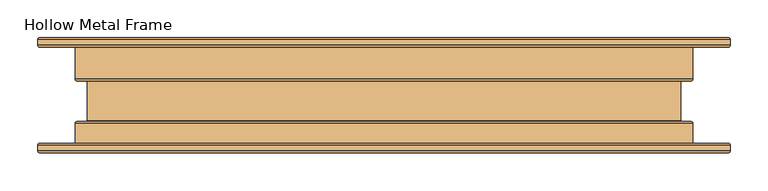
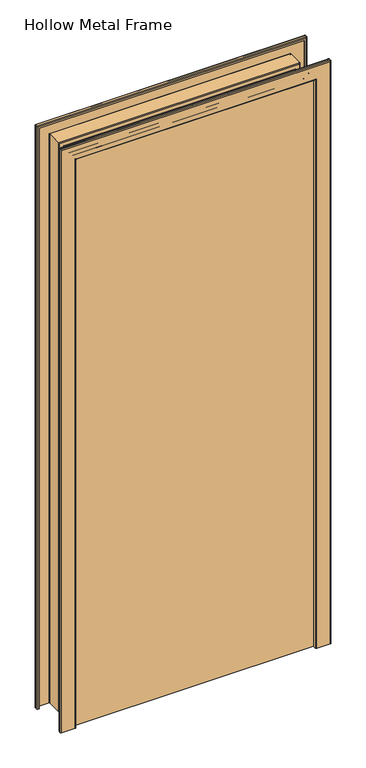
"""IFC4 building model written with IfcOpenShell, lengths in millimetres: door geometry, Hollow Metal Frame."""

import ifcopenshell
import ifcopenshell.guid

model = None  # the IFC model being written
_history = None  # IfcOwnerHistory: only IFC2X3 demands one
_inside = {}  # id of a spatial element -> (the spatial element, [elements in it])
_under = {}  # id of a project, library or spatial element -> (it, [spatial elements below it])
_declared = {}  # id of a project -> (the project, [libraries it declares])
_typed = {}  # id of a type object -> (the type object, [elements of that type])
_made_of = {}  # id of a material, layer set ... -> (it, [elements and type objects made of it])


def new_model(schema):
    """Start an empty IFC model of exactly this schema.

    Asked for "IFC4X3", IfcOpenShell would pick the latest addendum, in which some entities
    have other attributes; the version numbers below select the first issue.
    IFC2X3 requires an IfcOwnerHistory on every rooted entity: one is made here for all.
    """
    global model, _history
    if schema == "IFC4X3":
        model = ifcopenshell.file(schema_version=(4, 3, 0, 0))
    else:
        model = ifcopenshell.file(schema=schema)
    _inside.clear()
    _under.clear()
    _declared.clear()
    _typed.clear()
    _made_of.clear()
    _history = None
    if model.schema == "IFC2X3":
        org = make("IfcOrganization", Name="unknown")
        user = make(
            "IfcPersonAndOrganization",
            ThePerson=make("IfcPerson", FamilyName="unknown"),
            TheOrganization=org,
        )
        app = make(
            "IfcApplication",
            ApplicationDeveloper=org,
            Version="unknown",
            ApplicationFullName="unknown",
            ApplicationIdentifier="unknown",
        )
        _history = make(
            "IfcOwnerHistory",
            OwningUser=user,
            OwningApplication=app,
            ChangeAction="ADDED",
            CreationDate=0,
        )
    return model


def make(cls, **values):
    """One entity of the class cls with the attributes given. An attribute that is None is left unset."""
    return model.create_entity(
        cls, **{name: value for name, value in values.items() if value is not None}
    )


def rooted(cls, **values):
    """An entity with a GlobalId (a new one), such as an element, a storey or a relation."""
    return make(cls, GlobalId=ifcopenshell.guid.new(), OwnerHistory=_history, **values)


def si_unit(unit_type, name, prefix=None):
    """IfcSIUnit, for example si_unit("LENGTHUNIT", "METRE", prefix="MILLI")."""
    return make("IfcSIUnit", UnitType=unit_type, Prefix=prefix, Name=name)


def assignment(units):
    """IfcUnitAssignment: the units of a project."""
    return None if units is None else make("IfcUnitAssignment", Units=units)


def point(xyz):
    """IfcCartesianPoint."""
    return None if xyz is None else make("IfcCartesianPoint", Coordinates=xyz)


def direction(xyz):
    """IfcDirection."""
    return None if xyz is None else make("IfcDirection", DirectionRatios=xyz)


def frame(location, z_axis=None, x_axis=None):
    """IfcAxis2Placement3D, a coordinate frame: its origin and axes. An axis left out is left unset."""
    return make(
        "IfcAxis2Placement3D",
        Location=point(location),
        Axis=direction(z_axis),
        RefDirection=direction(x_axis),
    )


def origin():
    """The frame at (0, 0, 0) with its axes left unset."""
    return frame((0.0, 0.0, 0.0))


def origin_with_axes():
    """The frame at (0, 0, 0) with the z axis (0, 0, 1) and the x axis (1, 0, 0) written out."""
    return frame((0.0, 0.0, 0.0), z_axis=(0.0, 0.0, 1.0), x_axis=(1.0, 0.0, 0.0))


def place(relative_to, where):
    """IfcLocalPlacement: puts the frame where relative to a parent placement (None: the world)."""
    return make(
        "IfcLocalPlacement", PlacementRelTo=relative_to, RelativePlacement=where
    )


def context(
    kind, dimensions, precision=None, world=None, true_north=None, identifier=None
):
    """IfcGeometricRepresentationContext, for example the 3D "Model" context."""
    return make(
        "IfcGeometricRepresentationContext",
        ContextIdentifier=identifier,
        ContextType=kind,
        CoordinateSpaceDimension=dimensions,
        Precision=precision,
        WorldCoordinateSystem=world,
        TrueNorth=true_north,
    )


def project(units=None, contexts=None):
    """IfcProject with its units and contexts."""
    return rooted(
        "IfcProject",
        Name="project",
        RepresentationContexts=contexts,
        UnitsInContext=assignment(units),
    )


def spatial(cls, under=None, at=None, **own):
    """A site, building, storey or space (cls), placed at a placement, below another one or the project."""
    s = rooted(cls, ObjectPlacement=at, **own)
    if under is not None:
        _under.setdefault(under.id(), (under, []))[1].append(s)
    return s


def polyline(points):
    """IfcPolyline through the points."""
    return make("IfcPolyline", Points=[point(p) for p in points])


def circle_curve(where, radius):
    """IfcCircle in the frame where."""
    return make("IfcCircle", Position=where, Radius=radius)


def ellipse_curve(where, semi_axis1, semi_axis2):
    """IfcEllipse in the frame where."""
    return make(
        "IfcEllipse", Position=where, SemiAxis1=semi_axis1, SemiAxis2=semi_axis2
    )


def outline(outer, holes=None, kind="AREA"):
    """IfcArbitraryClosedProfileDef: a profile drawn as a closed curve; with holes, ...WithVoids."""
    if holes is None:
        return make("IfcArbitraryClosedProfileDef", ProfileType=kind, OuterCurve=outer)
    return make(
        "IfcArbitraryProfileDefWithVoids",
        ProfileType=kind,
        OuterCurve=outer,
        InnerCurves=holes,
    )


def extrude(swept, where, along, depth):
    """IfcExtrudedAreaSolid: the profile swept, set in the frame where, extruded along a direction by depth."""
    return make(
        "IfcExtrudedAreaSolid",
        SweptArea=swept,
        Position=where,
        ExtrudedDirection=direction(along),
        Depth=depth,
    )


def shape(context_of_items, identifier, shape_type, items):
    """IfcShapeRepresentation: the items that make up one representation, for example the "Body"."""
    return make(
        "IfcShapeRepresentation",
        ContextOfItems=context_of_items,
        RepresentationIdentifier=identifier,
        RepresentationType=shape_type,
        Items=items,
    )


def source(mapping_origin, context_of_items, identifier, shape_type, items):
    """IfcRepresentationMap: a shape defined once, which mapped items show again and again."""
    return make(
        "IfcRepresentationMap",
        MappingOrigin=mapping_origin,
        MappedRepresentation=shape(context_of_items, identifier, shape_type, items),
    )


def transform(
    local_origin,
    x_axis=None,
    y_axis=None,
    z_axis=None,
    scale=None,
    scale2=None,
    scale3=None,
    uniform=True,
):
    """IfcCartesianTransformationOperator3D, or its non-uniform kind. x_axis, y_axis, z_axis: its Axis1, 2, 3."""
    if uniform:
        return make(
            "IfcCartesianTransformationOperator3D",
            Axis1=direction(x_axis),
            Axis2=direction(y_axis),
            LocalOrigin=point(local_origin),
            Scale=scale,
            Axis3=direction(z_axis),
        )
    return make(
        "IfcCartesianTransformationOperator3DnonUniform",
        Axis1=direction(x_axis),
        Axis2=direction(y_axis),
        LocalOrigin=point(local_origin),
        Scale=scale,
        Axis3=direction(z_axis),
        Scale2=scale2,
        Scale3=scale3,
    )


def mapped(mapping_source, mapping_target):
    """IfcMappedItem: shows the shape of a source again, moved by a transform."""
    return make(
        "IfcMappedItem", MappingSource=mapping_source, MappingTarget=mapping_target
    )


def made_of(thing, what):
    """Note that an element or type object is made of a material, layer set ...; save() writes the relation."""
    if what is not None:
        _made_of.setdefault(what.id(), (what, []))[1].append(thing)
    return thing


def element(
    cls,
    number,
    at=None,
    inside=None,
    cuts=None,
    type_object=None,
    material=None,
    context=None,
    identifier="Body",
    shape_type=None,
    held_by="IfcProductDefinitionShape",
    body=None,
    shapes=None,
    **own,
):
    """One element of the class cls, such as IfcWall. Its Tag is "e" and its number.

    at: its placement. inside: the storey or other place that contains it. cuts: it is an
    opening in that element (IfcRelVoidsElement). A single representation is given by context,
    identifier, shape_type and body (its items); several are given by shapes. held_by: the class
    of the entity that holds the representations. save() writes the other relations.
    """
    e = rooted(cls, Tag="e%d" % number, ObjectPlacement=at, **own)
    if body is not None:
        shapes = [shape(context, identifier, shape_type, body)]
    if shapes is not None:
        e.Representation = make(held_by, Representations=shapes)
    if inside is not None:
        _inside.setdefault(inside.id(), (inside, []))[1].append(e)
    if cuts is not None:
        rooted(
            "IfcRelVoidsElement", RelatingBuildingElement=cuts, RelatedOpeningElement=e
        )
    if type_object is not None:
        _typed.setdefault(type_object.id(), (type_object, []))[1].append(e)
    return made_of(e, material)


def aggregate(whole, parts):
    """IfcRelAggregates: a whole, such as a stair, and the parts it consists of."""
    return rooted("IfcRelAggregates", RelatingObject=whole, RelatedObjects=parts)


def save(model, path):
    """Write the relations noted so far, then the file.

    IfcRelAggregates (storeys below a building ...), IfcRelContainedInSpatialStructure (elements
    in a storey), IfcRelDefinesByType, IfcRelAssociatesMaterial and IfcRelDeclares: one each for
    every whole, place, type object, material and project.
    """
    for whole, parts in _under.values():
        aggregate(whole, parts)
    for where, things in _inside.values():
        rooted(
            "IfcRelContainedInSpatialStructure",
            RelatedElements=things,
            RelatingStructure=where,
        )
    for kind, things in _typed.values():
        rooted("IfcRelDefinesByType", RelatedObjects=things, RelatingType=kind)
    for what, things in _made_of.values():
        rooted("IfcRelAssociatesMaterial", RelatedObjects=things, RelatingMaterial=what)
    for by, libraries in _declared.values():
        rooted("IfcRelDeclares", RelatingContext=by, RelatedDefinitions=libraries)
    model.write(path)


def plane_surface(at):
    """IfcPlane: the flat surface through the origin of the frame at, square to its z axis."""
    return make("IfcPlane", Position=at)


def cylinder_surface(at, radius):
    """IfcCylindricalSurface: all points at the distance radius from the z axis of the frame at."""
    return make("IfcCylindricalSurface", Position=at, Radius=radius)


def revolved_surface(curve, axis_point, axis_direction):
    """IfcSurfaceOfRevolution: the curve turned about the line through axis_point along axis_direction."""
    return make(
        "IfcSurfaceOfRevolution",
        SweptCurve=make("IfcArbitraryOpenProfileDef", ProfileType="CURVE", Curve=curve),
        AxisPosition=make("IfcAxis1Placement", Location=point(axis_point), Axis=direction(axis_direction)),
    )


def advanced_brep(points, edges, surfaces, faces):
    """IfcAdvancedBrep: a solid bounded by faces that lie on surfaces and meet in shared edges.

    An edge is (start, end): straight between two places in points (the first is 0);
    or (start, end, curve); or (start, end, curve, False) where it runs against its curve.
    A face is (place in surfaces, loops), or (place, loops, False) where it looks against
    its surface's normal. A loop lists edges by number (the first is 1), with a minus sign
    where the edge is run from its end to its start. The first loop is the outer one.
    """
    corners = [point(p) for p in points]
    vertices = [make("IfcVertexPoint", VertexGeometry=c) for c in corners]
    made = []
    for start, end, *more in edges:
        made.append(
            make(
                "IfcEdgeCurve",
                EdgeStart=vertices[start],
                EdgeEnd=vertices[end],
                EdgeGeometry=more[0] if more else make("IfcPolyline", Points=[corners[start], corners[end]]),
                SameSense=more[1] if len(more) > 1 else True,
            )
        )
    hull = []
    for where, loops, *sense in faces:
        bounds = []
        for j, loop in enumerate(loops):
            ring = [make("IfcOrientedEdge", EdgeElement=made[abs(k) - 1], Orientation=k > 0) for k in loop]
            bounds.append(
                make(
                    "IfcFaceOuterBound" if j == 0 else "IfcFaceBound",
                    Bound=make("IfcEdgeLoop", EdgeList=ring),
                    Orientation=True,
                )
            )
        hull.append(make("IfcAdvancedFace", Bounds=bounds, FaceSurface=surfaces[where], SameSense=sense[0] if sense else True))
    return make("IfcAdvancedBrep", Outer=make("IfcClosedShell", CfsFaces=hull))


def hollow_metal_frame_ca3e70b1(model_context):
    return source(origin(), model_context, "Body", "SolidModel", [
        advanced_brep(
        [(-454.62825, 63.5635, 0.0), (-457.2, 66.13525, 0.0), (-457.2, 73.66, 0.0), (-454.62825, 76.23175, 0.0), (-408.97175, 76.23175, 0.0), (-406.4, 73.66, 0.0), (-406.4, 21.68525, 0.0), (-405.384, 20.66925, 0.0), (-393.09675, 20.66925, 0.0), (-390.525, 18.0975, 0.0), (-390.525, -33.6931, 0.0), (-393.09675, -36.26485, 0.0), (-405.384, -36.26485, 0.0), (-406.4, -37.28085, 0.0), (-406.4, -73.5965, 0.0), (-408.97175, -76.16825, 0.0), (-454.62825, -76.16825, 0.0), (-457.2, -73.5965, 0.0), (-457.2, -66.07175, 0.0), (-454.62825, -63.5, 0.0), (-449.2625, -63.5, 0.0), (-449.2625, -65.05575, 0.0), (-454.62825, -65.05575, 0.0), (-455.64425, -66.07175, 0.0), (-455.64425, -73.5965, 0.0), (-454.62825, -74.6125, 0.0), (-408.97175, -74.6125, 0.0), (-407.95575, -73.5965, 0.0), (-407.95575, -37.28085, 0.0), (-405.384, -34.7091, 0.0), (-393.09675, -34.7091, 0.0), (-392.08075, -33.6931, 0.0), (-392.08075, 18.0975, 0.0), (-393.09675, 19.1135, 0.0), (-405.384, 19.1135, 0.0), (-407.95575, 21.68525, 0.0), (-407.95575, 73.66, 0.0), (-408.97175, 74.676, 0.0), (-454.62825, 74.676, 0.0), (-455.64425, 73.66, 0.0), (-455.64425, 66.13525, 0.0), (-454.62825, 65.11925, 0.0), (-449.2625, 65.11925, 0.0), (-449.2625, 63.5635, 0.0), (-454.62825, 63.5635, 2080.2282501), (-457.2, 66.13525, 2082.8000001), (-457.2, 73.66, 2082.8000001), (-454.62825, 76.23175, 2080.2282501), (454.62825, 76.23175, 2080.2282501), (454.62825, 76.23175, 0.0), (408.97175, 76.23175, 0.0), (408.97175, 76.23175, 2034.5717501), (-408.97175, 76.23175, 2034.5717501), (-406.4, 73.66, 2032.0000001), (-406.4, 21.68525, 2032.0000001), (-405.384, 20.66925, 2030.9840001), (405.384, 20.66925, 2030.9840001), (405.384, 20.66925, 0.0), (393.09675, 20.66925, 0.0), (393.09675, 20.66925, 2018.6967501), (-393.09675, 20.66925, 2018.6967501), (-390.525, 18.0975, 2016.1250001), (-390.525, -33.6931, 2016.1250001), (-393.09675, -36.26485, 2018.6967501), (393.09675, -36.26485, 2018.6967501), (393.09675, -36.26485, 0.0), (405.384, -36.26485, 0.0), (405.384, -36.26485, 2030.9840001), (-405.384, -36.26485, 2030.9840001), (-406.4, -37.28085, 2032.0000001), (-406.4, -73.5965, 2032.0000001), (-408.97175, -76.16825, 2034.5717501), (408.97175, -76.16825, 2034.5717501), (408.97175, -76.16825, 0.0), (454.62825, -76.16825, 0.0), (454.62825, -76.16825, 2080.2282501), (-454.62825, -76.16825, 2080.2282501), (-457.2, -73.5965, 2082.8000001), (-457.2, -66.07175, 2082.8000001), (-454.62825, -63.5, 2080.2282501), (454.62825, -63.5, 2080.2282501), (454.62825, -63.5, 0.0), (449.2625, -63.5, 0.0), (449.2625, -63.5, 2074.8625001), (-449.2625, -63.5, 2074.8625001), (-449.2625, -65.05575, 2074.8625001), (449.2625, -65.05575, 2074.8625001), (449.2625, -65.05575, 0.0), (454.62825, -65.05575, 0.0), (454.62825, -65.05575, 2080.2282501), (-454.62825, -65.05575, 2080.2282501), (-455.64425, -66.07175, 2081.2442501), (-455.64425, -73.5965, 2081.2442501), (-454.62825, -74.6125, 2080.2282501), (454.62825, -74.6125, 2080.2282501), (454.62825, -74.6125, 0.0), (408.97175, -74.6125, 0.0), (408.97175, -74.6125, 2034.5717501), (-408.97175, -74.6125, 2034.5717501), (-407.95575, -73.5965, 2033.5557501), (-407.95575, -37.28085, 2033.5557501), (-405.384, -34.7091, 2030.9840001), (405.384, -34.7091, 2030.9840001), (405.384, -34.7091, 0.0), (393.09675, -34.7091, 0.0), (393.09675, -34.7091, 2018.6967501), (-393.09675, -34.7091, 2018.6967501), (-392.08075, -33.6931, 2017.6807501), (-392.08075, 18.0975, 2017.6807501), (-393.09675, 19.1135, 2018.6967501), (393.09675, 19.1135, 2018.6967501), (393.09675, 19.1135, 0.0), (405.384, 19.1135, 0.0), (405.384, 19.1135, 2030.9840001), (-405.384, 19.1135, 2030.9840001), (-407.95575, 21.68525, 2033.5557501), (-407.95575, 73.66, 2033.5557501), (-408.97175, 74.676, 2034.5717501), (408.97175, 74.676, 2034.5717501), (408.97175, 74.676, 0.0), (454.62825, 74.676, 0.0), (454.62825, 74.676, 2080.2282501), (-454.62825, 74.676, 2080.2282501), (-455.64425, 73.66, 2081.2442501), (-455.64425, 66.13525, 2081.2442501), (-454.62825, 65.11925, 2080.2282501), (454.62825, 65.11925, 2080.2282501), (454.62825, 65.11925, 0.0), (449.2625, 65.11925, 0.0), (449.2625, 65.11925, 2074.8625001), (-449.2625, 65.11925, 2074.8625001), (-449.2625, 63.5635, 2074.8625001), (449.2625, 63.5635, 2074.8625001), (449.2625, 63.5635, 0.0), (454.62825, 63.5635, 0.0), (454.62825, 63.5635, 2080.2282501), (457.2, 66.13525, 2082.8000001), (457.2, 73.66, 2082.8000001), (406.4, 73.66, 2032.0000001), (406.4, 21.68525, 2032.0000001), (390.525, 18.0975, 2016.1250001), (390.525, -33.6931, 2016.1250001), (406.4, -37.28085, 2032.0000001), (406.4, -73.5965, 2032.0000001), (457.2, -73.5965, 2082.8000001), (457.2, -66.07175, 2082.8000001), (455.64425, -66.07175, 2081.2442501), (455.64425, -73.5965, 2081.2442501), (407.95575, -73.5965, 2033.5557501), (407.95575, -37.28085, 2033.5557501), (392.08075, -33.6931, 2017.6807501), (392.08075, 18.0975, 2017.6807501), (407.95575, 21.68525, 2033.5557501), (407.95575, 73.66, 2033.5557501), (455.64425, 73.66, 2081.2442501), (455.64425, 66.13525, 2081.2442501), (455.64425, 66.13525, 0.0), (455.64425, 73.66, 0.0), (407.95575, 73.66, 0.0), (407.95575, 21.68525, 0.0), (392.08075, 18.0975, 0.0), (392.08075, -33.6931, 0.0), (407.95575, -37.28085, 0.0), (407.95575, -73.5965, 0.0), (455.64425, -73.5965, 0.0), (455.64425, -66.07175, 0.0), (457.2, -66.07175, 0.0), (457.2, -73.5965, 0.0), (406.4, -73.5965, 0.0), (406.4, -37.28085, 0.0), (390.525, -33.6931, 0.0), (390.525, 18.0975, 0.0), (406.4, 21.68525, 0.0), (406.4, 73.66, 0.0), (457.2, 73.66, 0.0), (457.2, 66.13525, 0.0)],
        [
            (0, 1, circle_curve(frame((-454.62825, 66.13525, 0.0), z_axis=(0.0, 0.0, -1.0), x_axis=(0.0, -1.0, 0.0)), 2.57175)),
            (1, 2),
            (2, 3, circle_curve(frame((-454.62825, 73.66, 0.0), z_axis=(0.0, 0.0, -1.0), x_axis=(0.0, -1.0, 0.0)), 2.57175)),
            (3, 4),
            (4, 5, circle_curve(frame((-408.97175, 73.66, 0.0), z_axis=(0.0, 0.0, -1.0), x_axis=(0.0, -1.0, 0.0)), 2.57175)),
            (5, 6),
            (6, 7, circle_curve(frame((-405.384, 21.68525, 0.0), z_axis=(0.0, 0.0, 1.0), x_axis=(0.0, -1.0, 0.0)), 1.016)),
            (7, 8),
            (8, 9, circle_curve(frame((-393.09675, 18.0975, 0.0), z_axis=(0.0, 0.0, -1.0), x_axis=(0.0, -1.0, 0.0)), 2.57175)),
            (9, 10),
            (10, 11, circle_curve(frame((-393.09675, -33.6931, 0.0), z_axis=(0.0, 0.0, -1.0), x_axis=(0.0, -1.0, 0.0)), 2.57175)),
            (11, 12),
            (12, 13, circle_curve(frame((-405.384, -37.28085, 0.0), z_axis=(0.0, 0.0, 1.0), x_axis=(0.0, -1.0, 0.0)), 1.016)),
            (13, 14),
            (14, 15, circle_curve(frame((-408.97175, -73.5965, 0.0), z_axis=(0.0, 0.0, -1.0), x_axis=(0.0, -1.0, 0.0)), 2.57175)),
            (15, 16),
            (16, 17, circle_curve(frame((-454.62825, -73.5965, 0.0), z_axis=(0.0, 0.0, -1.0), x_axis=(0.0, -1.0, 0.0)), 2.57175)),
            (17, 18),
            (18, 19, circle_curve(frame((-454.62825, -66.07175, 0.0), z_axis=(0.0, 0.0, -1.0), x_axis=(0.0, -1.0, 0.0)), 2.57175)),
            (19, 20),
            (20, 21),
            (21, 22),
            (22, 23, circle_curve(frame((-454.62825, -66.07175, 0.0), z_axis=(0.0, 0.0, 1.0), x_axis=(0.0, -1.0, 0.0)), 1.016)),
            (23, 24),
            (24, 25, circle_curve(frame((-454.62825, -73.5965, 0.0), z_axis=(0.0, 0.0, 1.0), x_axis=(0.0, -1.0, 0.0)), 1.016)),
            (25, 26),
            (26, 27, circle_curve(frame((-408.97175, -73.5965, 0.0), z_axis=(0.0, 0.0, 1.0), x_axis=(0.0, -1.0, 0.0)), 1.016)),
            (27, 28),
            (28, 29, circle_curve(frame((-405.384, -37.28085, 0.0), z_axis=(0.0, 0.0, -1.0), x_axis=(0.0, -1.0, 0.0)), 2.57175)),
            (29, 30),
            (30, 31, circle_curve(frame((-393.09675, -33.6931, 0.0), z_axis=(0.0, 0.0, 1.0), x_axis=(0.0, -1.0, 0.0)), 1.016)),
            (31, 32),
            (32, 33, circle_curve(frame((-393.09675, 18.0975, 0.0), z_axis=(0.0, 0.0, 1.0), x_axis=(0.0, -1.0, 0.0)), 1.016)),
            (33, 34),
            (34, 35, circle_curve(frame((-405.384, 21.68525, 0.0), z_axis=(0.0, 0.0, -1.0), x_axis=(0.0, -1.0, 0.0)), 2.57175)),
            (35, 36),
            (36, 37, circle_curve(frame((-408.97175, 73.66, 0.0), z_axis=(0.0, 0.0, 1.0), x_axis=(0.0, -1.0, 0.0)), 1.016)),
            (37, 38),
            (38, 39, circle_curve(frame((-454.62825, 73.66, 0.0), z_axis=(0.0, 0.0, 1.0), x_axis=(0.0, -1.0, 0.0)), 1.016)),
            (39, 40),
            (40, 41, circle_curve(frame((-454.62825, 66.13525, 0.0), z_axis=(0.0, 0.0, 1.0), x_axis=(0.0, -1.0, 0.0)), 1.016)),
            (41, 42),
            (42, 43),
            (43, 0),
            (0, 44),
            (44, 45, ellipse_curve(frame((-454.62825, 66.13525, 2080.2282501), z_axis=(-0.7071067811865475, 0.0, -0.7071067811865475), x_axis=(0.7071067811865474, 0.0, -0.7071067811865476)), 3.6370037, 2.57175)),
            (45, 1),
            (45, 46),
            (46, 2),
            (46, 47, ellipse_curve(frame((-454.62825, 73.66, 2080.2282501), z_axis=(-0.7071067811865475, 0.0, -0.7071067811865475), x_axis=(0.7071067811865474, 0.0, -0.7071067811865476)), 3.6370037, 2.57175)),
            (47, 3),
            (47, 48),
            (48, 49),
            (49, 50),
            (50, 51),
            (51, 52),
            (52, 4),
            (52, 53, ellipse_curve(frame((-408.97175, 73.66, 2034.5717501), z_axis=(-0.7071067811865475, 0.0, -0.7071067811865475), x_axis=(0.7071067811865474, 0.0, -0.7071067811865476)), 3.6370037, 2.57175)),
            (53, 5),
            (53, 54),
            (54, 6),
            (54, 55, ellipse_curve(frame((-405.384, 21.68525, 2030.9840001), z_axis=(0.7071067811865475, 0.0, 0.7071067811865475), x_axis=(-0.7071067811865474, 0.0, 0.7071067811865476)), 1.436841, 1.016)),
            (55, 7),
            (55, 56),
            (56, 57),
            (57, 58),
            (58, 59),
            (59, 60),
            (60, 8),
            (60, 61, ellipse_curve(frame((-393.09675, 18.0975, 2018.6967501), z_axis=(-0.7071067811865475, 0.0, -0.7071067811865475), x_axis=(0.7071067811865474, 0.0, -0.7071067811865476)), 3.6370037, 2.57175)),
            (61, 9),
            (61, 62),
            (62, 10),
            (62, 63, ellipse_curve(frame((-393.09675, -33.6931, 2018.6967501), z_axis=(-0.7071067811865475, 0.0, -0.7071067811865475), x_axis=(0.7071067811865474, 0.0, -0.7071067811865476)), 3.6370037, 2.57175)),
            (63, 11),
            (63, 64),
            (64, 65),
            (65, 66),
            (66, 67),
            (67, 68),
            (68, 12),
            (68, 69, ellipse_curve(frame((-405.384, -37.28085, 2030.9840001), z_axis=(0.7071067811865475, 0.0, 0.7071067811865475), x_axis=(-0.7071067811865474, 0.0, 0.7071067811865476)), 1.436841, 1.016)),
            (69, 13),
            (69, 70),
            (70, 14),
            (70, 71, ellipse_curve(frame((-408.97175, -73.5965, 2034.5717501), z_axis=(-0.7071067811865475, 0.0, -0.7071067811865475), x_axis=(0.7071067811865474, 0.0, -0.7071067811865476)), 3.6370037, 2.57175)),
            (71, 15),
            (71, 72),
            (72, 73),
            (73, 74),
            (74, 75),
            (75, 76),
            (76, 16),
            (76, 77, ellipse_curve(frame((-454.62825, -73.5965, 2080.2282501), z_axis=(-0.7071067811865475, 0.0, -0.7071067811865475), x_axis=(0.7071067811865474, 0.0, -0.7071067811865476)), 3.6370037, 2.57175)),
            (77, 17),
            (77, 78),
            (78, 18),
            (78, 79, ellipse_curve(frame((-454.62825, -66.07175, 2080.2282501), z_axis=(-0.7071067811865475, 0.0, -0.7071067811865475), x_axis=(0.7071067811865474, 0.0, -0.7071067811865476)), 3.6370037, 2.57175)),
            (79, 19),
            (79, 80),
            (80, 81),
            (81, 82),
            (82, 83),
            (83, 84),
            (84, 20),
            (84, 85),
            (85, 21),
            (85, 86),
            (86, 87),
            (87, 88),
            (88, 89),
            (89, 90),
            (90, 22),
            (90, 91, ellipse_curve(frame((-454.62825, -66.07175, 2080.2282501), z_axis=(0.7071067811865475, 0.0, 0.7071067811865475), x_axis=(-0.7071067811865474, 0.0, 0.7071067811865476)), 1.436841, 1.016)),
            (91, 23),
            (91, 92),
            (92, 24),
            (92, 93, ellipse_curve(frame((-454.62825, -73.5965, 2080.2282501), z_axis=(0.7071067811865475, 0.0, 0.7071067811865475), x_axis=(-0.7071067811865474, 0.0, 0.7071067811865476)), 1.436841, 1.016)),
            (93, 25),
            (93, 94),
            (94, 95),
            (95, 96),
            (96, 97),
            (97, 98),
            (98, 26),
            (98, 99, ellipse_curve(frame((-408.97175, -73.5965, 2034.5717501), z_axis=(0.7071067811865475, 0.0, 0.7071067811865475), x_axis=(-0.7071067811865474, 0.0, 0.7071067811865476)), 1.436841, 1.016)),
            (99, 27),
            (99, 100),
            (100, 28),
            (100, 101, ellipse_curve(frame((-405.384, -37.28085, 2030.9840001), z_axis=(-0.7071067811865475, 0.0, -0.7071067811865475), x_axis=(0.7071067811865474, 0.0, -0.7071067811865476)), 3.6370037, 2.57175)),
            (101, 29),
            (101, 102),
            (102, 103),
            (103, 104),
            (104, 105),
            (105, 106),
            (106, 30),
            (106, 107, ellipse_curve(frame((-393.09675, -33.6931, 2018.6967501), z_axis=(0.7071067811865475, 0.0, 0.7071067811865475), x_axis=(-0.7071067811865474, 0.0, 0.7071067811865476)), 1.436841, 1.016)),
            (107, 31),
            (107, 108),
            (108, 32),
            (108, 109, ellipse_curve(frame((-393.09675, 18.0975, 2018.6967501), z_axis=(0.7071067811865475, 0.0, 0.7071067811865475), x_axis=(-0.7071067811865474, 0.0, 0.7071067811865476)), 1.436841, 1.016)),
            (109, 33),
            (109, 110),
            (110, 111),
            (111, 112),
            (112, 113),
            (113, 114),
            (114, 34),
            (114, 115, ellipse_curve(frame((-405.384, 21.68525, 2030.9840001), z_axis=(-0.7071067811865475, 0.0, -0.7071067811865475), x_axis=(0.7071067811865474, 0.0, -0.7071067811865476)), 3.6370037, 2.57175)),
            (115, 35),
            (115, 116),
            (116, 36),
            (116, 117, ellipse_curve(frame((-408.97175, 73.66, 2034.5717501), z_axis=(0.7071067811865475, 0.0, 0.7071067811865475), x_axis=(-0.7071067811865474, 0.0, 0.7071067811865476)), 1.436841, 1.016)),
            (117, 37),
            (117, 118),
            (118, 119),
            (119, 120),
            (120, 121),
            (121, 122),
            (122, 38),
            (122, 123, ellipse_curve(frame((-454.62825, 73.66, 2080.2282501), z_axis=(0.7071067811865475, 0.0, 0.7071067811865475), x_axis=(-0.7071067811865474, 0.0, 0.7071067811865476)), 1.436841, 1.016)),
            (123, 39),
            (123, 124),
            (124, 40),
            (124, 125, ellipse_curve(frame((-454.62825, 66.13525, 2080.2282501), z_axis=(0.7071067811865475, 0.0, 0.7071067811865475), x_axis=(-0.7071067811865474, 0.0, 0.7071067811865476)), 1.436841, 1.016)),
            (125, 41),
            (125, 126),
            (126, 127),
            (127, 128),
            (128, 129),
            (129, 130),
            (130, 42),
            (130, 131),
            (131, 43),
            (131, 132),
            (132, 133),
            (133, 134),
            (134, 135),
            (135, 44),
            (135, 136, ellipse_curve(frame((454.62825, 66.13525, 2080.2282501), z_axis=(-0.7071067811865475, 0.0, 0.7071067811865475), x_axis=(-0.7071067811865476, 0.0, -0.7071067811865474)), 3.6370037, 2.57175)),
            (136, 45),
            (136, 137),
            (137, 46),
            (137, 48, ellipse_curve(frame((454.62825, 73.66, 2080.2282501), z_axis=(-0.7071067811865475, 0.0, 0.7071067811865475), x_axis=(-0.7071067811865476, 0.0, -0.7071067811865474)), 3.6370037, 2.57175)),
            (51, 138, ellipse_curve(frame((408.97175, 73.66, 2034.5717501), z_axis=(-0.7071067811865475, 0.0, 0.7071067811865475), x_axis=(-0.7071067811865476, 0.0, -0.7071067811865474)), 3.6370037, 2.57175)),
            (138, 53),
            (138, 139),
            (139, 54),
            (139, 56, ellipse_curve(frame((405.384, 21.68525, 2030.9840001), z_axis=(0.7071067811865475, 0.0, -0.7071067811865475), x_axis=(0.7071067811865476, 0.0, 0.7071067811865474)), 1.436841, 1.016)),
            (59, 140, ellipse_curve(frame((393.09675, 18.0975, 2018.6967501), z_axis=(-0.7071067811865475, 0.0, 0.7071067811865475), x_axis=(-0.7071067811865476, 0.0, -0.7071067811865474)), 3.6370037, 2.57175)),
            (140, 61),
            (140, 141),
            (141, 62),
            (141, 64, ellipse_curve(frame((393.09675, -33.6931, 2018.6967501), z_axis=(-0.7071067811865475, 0.0, 0.7071067811865475), x_axis=(-0.7071067811865476, 0.0, -0.7071067811865474)), 3.6370037, 2.57175)),
            (67, 142, ellipse_curve(frame((405.384, -37.28085, 2030.9840001), z_axis=(0.7071067811865475, 0.0, -0.7071067811865475), x_axis=(0.7071067811865476, 0.0, 0.7071067811865474)), 1.436841, 1.016)),
            (142, 69),
            (142, 143),
            (143, 70),
            (143, 72, ellipse_curve(frame((408.97175, -73.5965, 2034.5717501), z_axis=(-0.7071067811865475, 0.0, 0.7071067811865475), x_axis=(-0.7071067811865476, 0.0, -0.7071067811865474)), 3.6370037, 2.57175)),
            (75, 144, ellipse_curve(frame((454.62825, -73.5965, 2080.2282501), z_axis=(-0.7071067811865475, 0.0, 0.7071067811865475), x_axis=(-0.7071067811865476, 0.0, -0.7071067811865474)), 3.6370037, 2.57175)),
            (144, 77),
            (144, 145),
            (145, 78),
            (145, 80, ellipse_curve(frame((454.62825, -66.07175, 2080.2282501), z_axis=(-0.7071067811865475, 0.0, 0.7071067811865475), x_axis=(-0.7071067811865476, 0.0, -0.7071067811865474)), 3.6370037, 2.57175)),
            (83, 86),
            (89, 146, ellipse_curve(frame((454.62825, -66.07175, 2080.2282501), z_axis=(0.7071067811865475, 0.0, -0.7071067811865475), x_axis=(0.7071067811865476, 0.0, 0.7071067811865474)), 1.436841, 1.016)),
            (146, 91),
            (146, 147),
            (147, 92),
            (147, 94, ellipse_curve(frame((454.62825, -73.5965, 2080.2282501), z_axis=(0.7071067811865475, 0.0, -0.7071067811865475), x_axis=(0.7071067811865476, 0.0, 0.7071067811865474)), 1.436841, 1.016)),
            (97, 148, ellipse_curve(frame((408.97175, -73.5965, 2034.5717501), z_axis=(0.7071067811865475, 0.0, -0.7071067811865475), x_axis=(0.7071067811865476, 0.0, 0.7071067811865474)), 1.436841, 1.016)),
            (148, 99),
            (148, 149),
            (149, 100),
            (149, 102, ellipse_curve(frame((405.384, -37.28085, 2030.9840001), z_axis=(-0.7071067811865475, 0.0, 0.7071067811865475), x_axis=(-0.7071067811865476, 0.0, -0.7071067811865474)), 3.6370037, 2.57175)),
            (105, 150, ellipse_curve(frame((393.09675, -33.6931, 2018.6967501), z_axis=(0.7071067811865475, 0.0, -0.7071067811865475), x_axis=(0.7071067811865476, 0.0, 0.7071067811865474)), 1.436841, 1.016)),
            (150, 107),
            (150, 151),
            (151, 108),
            (151, 110, ellipse_curve(frame((393.09675, 18.0975, 2018.6967501), z_axis=(0.7071067811865475, 0.0, -0.7071067811865475), x_axis=(0.7071067811865476, 0.0, 0.7071067811865474)), 1.436841, 1.016)),
            (113, 152, ellipse_curve(frame((405.384, 21.68525, 2030.9840001), z_axis=(-0.7071067811865475, 0.0, 0.7071067811865475), x_axis=(-0.7071067811865476, 0.0, -0.7071067811865474)), 3.6370037, 2.57175)),
            (152, 115),
            (152, 153),
            (153, 116),
            (153, 118, ellipse_curve(frame((408.97175, 73.66, 2034.5717501), z_axis=(0.7071067811865475, 0.0, -0.7071067811865475), x_axis=(0.7071067811865476, 0.0, 0.7071067811865474)), 1.436841, 1.016)),
            (121, 154, ellipse_curve(frame((454.62825, 73.66, 2080.2282501), z_axis=(0.7071067811865475, 0.0, -0.7071067811865475), x_axis=(0.7071067811865476, 0.0, 0.7071067811865474)), 1.436841, 1.016)),
            (154, 123),
            (154, 155),
            (155, 124),
            (155, 126, ellipse_curve(frame((454.62825, 66.13525, 2080.2282501), z_axis=(0.7071067811865475, 0.0, -0.7071067811865475), x_axis=(0.7071067811865476, 0.0, 0.7071067811865474)), 1.436841, 1.016)),
            (129, 132),
            (133, 128),
            (127, 156, circle_curve(frame((454.62825, 66.13525, 0.0), z_axis=(0.0, 0.0, 1.0), x_axis=(0.0, -1.0, 0.0)), 1.016)),
            (156, 157),
            (157, 120, circle_curve(frame((454.62825, 73.66, 0.0), z_axis=(0.0, 0.0, 1.0), x_axis=(0.0, -1.0, 0.0)), 1.016)),
            (119, 158, circle_curve(frame((408.97175, 73.66, 0.0), z_axis=(0.0, 0.0, 1.0), x_axis=(0.0, -1.0, 0.0)), 1.016)),
            (158, 159),
            (159, 112, circle_curve(frame((405.384, 21.68525, 0.0), z_axis=(0.0, 0.0, -1.0), x_axis=(0.0, -1.0, 0.0)), 2.57175)),
            (111, 160, circle_curve(frame((393.09675, 18.0975, 0.0), z_axis=(0.0, 0.0, 1.0), x_axis=(0.0, -1.0, 0.0)), 1.016)),
            (160, 161),
            (161, 104, circle_curve(frame((393.09675, -33.6931, 0.0), z_axis=(0.0, 0.0, 1.0), x_axis=(0.0, -1.0, 0.0)), 1.016)),
            (103, 162, circle_curve(frame((405.384, -37.28085, 0.0), z_axis=(0.0, 0.0, -1.0), x_axis=(0.0, -1.0, 0.0)), 2.57175)),
            (162, 163),
            (163, 96, circle_curve(frame((408.97175, -73.5965, 0.0), z_axis=(0.0, 0.0, 1.0), x_axis=(0.0, -1.0, 0.0)), 1.016)),
            (95, 164, circle_curve(frame((454.62825, -73.5965, 0.0), z_axis=(0.0, 0.0, 1.0), x_axis=(0.0, -1.0, 0.0)), 1.016)),
            (164, 165),
            (165, 88, circle_curve(frame((454.62825, -66.07175, 0.0), z_axis=(0.0, 0.0, 1.0), x_axis=(0.0, -1.0, 0.0)), 1.016)),
            (87, 82),
            (81, 166, circle_curve(frame((454.62825, -66.07175, 0.0), z_axis=(0.0, 0.0, -1.0), x_axis=(0.0, -1.0, 0.0)), 2.57175)),
            (166, 167),
            (167, 74, circle_curve(frame((454.62825, -73.5965, 0.0), z_axis=(0.0, 0.0, -1.0), x_axis=(0.0, -1.0, 0.0)), 2.57175)),
            (73, 168, circle_curve(frame((408.97175, -73.5965, 0.0), z_axis=(0.0, 0.0, -1.0), x_axis=(0.0, -1.0, 0.0)), 2.57175)),
            (168, 169),
            (169, 66, circle_curve(frame((405.384, -37.28085, 0.0), z_axis=(0.0, 0.0, 1.0), x_axis=(0.0, -1.0, 0.0)), 1.016)),
            (65, 170, circle_curve(frame((393.09675, -33.6931, 0.0), z_axis=(0.0, 0.0, -1.0), x_axis=(0.0, -1.0, 0.0)), 2.57175)),
            (170, 171),
            (171, 58, circle_curve(frame((393.09675, 18.0975, 0.0), z_axis=(0.0, 0.0, -1.0), x_axis=(0.0, -1.0, 0.0)), 2.57175)),
            (57, 172, circle_curve(frame((405.384, 21.68525, 0.0), z_axis=(0.0, 0.0, 1.0), x_axis=(0.0, -1.0, 0.0)), 1.016)),
            (172, 173),
            (173, 50, circle_curve(frame((408.97175, 73.66, 0.0), z_axis=(0.0, 0.0, -1.0), x_axis=(0.0, -1.0, 0.0)), 2.57175)),
            (49, 174, circle_curve(frame((454.62825, 73.66, 0.0), z_axis=(0.0, 0.0, -1.0), x_axis=(0.0, -1.0, 0.0)), 2.57175)),
            (174, 175),
            (175, 134, circle_curve(frame((454.62825, 66.13525, 0.0), z_axis=(0.0, 0.0, -1.0), x_axis=(0.0, -1.0, 0.0)), 2.57175)),
            (175, 136),
            (174, 137),
            (173, 138),
            (172, 139),
            (171, 140),
            (170, 141),
            (169, 142),
            (168, 143),
            (167, 144),
            (166, 145),
            (165, 146),
            (164, 147),
            (163, 148),
            (162, 149),
            (161, 150),
            (160, 151),
            (159, 152),
            (158, 153),
            (157, 154),
            (156, 155),
        ],
        [
            plane_surface(frame((-417.5125, -63.5, 0.0), z_axis=(0.0, 0.0, -1.0), x_axis=(1.0, 0.0, 0.0))),
            cylinder_surface(frame((-454.62825, 66.13525, 0.0), z_axis=(0.0, 0.0, -1.0), x_axis=(0.0, -1.0, 0.0)), 2.57175),
            plane_surface(frame((-457.2, 66.13525, 0.0), z_axis=(-1.0, 0.0, 0.0), x_axis=(0.0, 0.0, 1.0))),
            cylinder_surface(frame((-454.62825, 73.66, 0.0), z_axis=(0.0, 0.0, -1.0), x_axis=(0.0, -1.0, 0.0)), 2.57175),
            plane_surface(frame((-454.62825, 76.23175, 0.0), z_axis=(0.0, 1.0, 0.0), x_axis=(0.0, 0.0, 1.0))),
            cylinder_surface(frame((-408.97175, 73.66, 0.0), z_axis=(0.0, 0.0, -1.0), x_axis=(0.0, -1.0, 0.0)), 2.57175),
            plane_surface(frame((-406.4, 73.66, 0.0), z_axis=(1.0, 0.0, 0.0), x_axis=(0.0, 0.0, 1.0))),
            revolved_surface(polyline([(-405.384, 20.669249999999998, 2032.0000001145868), (-405.384, 20.669249999999998, 0.0)]), (-405.384, 21.68525, 0.0), (0.0, 0.0, 1.0)),
            plane_surface(frame((-405.384, 20.66925, 0.0), z_axis=(0.0, 1.0, 0.0), x_axis=(0.0, 0.0, 1.0))),
            cylinder_surface(frame((-393.09675, 18.0975, 0.0), z_axis=(0.0, 0.0, -1.0), x_axis=(0.0, -1.0, 0.0)), 2.57175),
            plane_surface(frame((-390.525, 18.0975, 0.0), z_axis=(1.0, 0.0, 0.0), x_axis=(0.0, 0.0, 1.0))),
            cylinder_surface(frame((-393.09675, -33.6931, 0.0), z_axis=(0.0, 0.0, -1.0), x_axis=(0.0, -1.0, 0.0)), 2.57175),
            plane_surface(frame((-393.09675, -36.26485, 0.0), z_axis=(0.0, -1.0, 0.0), x_axis=(0.0, 0.0, 1.0))),
            revolved_surface(polyline([(-405.384, -38.29685, 2032.0000001145868), (-405.384, -38.29685, 0.0)]), (-405.384, -37.28085, 0.0), (0.0, 0.0, 1.0)),
            plane_surface(frame((-406.4, -37.28085, 0.0), z_axis=(1.0, 0.0, 0.0), x_axis=(0.0, 0.0, 1.0))),
            cylinder_surface(frame((-408.97175, -73.5965, 0.0), z_axis=(0.0, 0.0, -1.0), x_axis=(0.0, -1.0, 0.0)), 2.57175),
            plane_surface(frame((-408.97175, -76.16825, 0.0), z_axis=(0.0, -1.0, 0.0), x_axis=(0.0, 0.0, 1.0))),
            cylinder_surface(frame((-454.62825, -73.5965, 0.0), z_axis=(0.0, 0.0, -1.0), x_axis=(0.0, -1.0, 0.0)), 2.57175),
            plane_surface(frame((-457.2, -73.5965, 0.0), z_axis=(-1.0, 0.0, 0.0), x_axis=(0.0, 0.0, 1.0))),
            cylinder_surface(frame((-454.62825, -66.07175, 0.0), z_axis=(0.0, 0.0, -1.0), x_axis=(0.0, -1.0, 0.0)), 2.57175),
            plane_surface(frame((-454.62825, -63.5, 0.0), z_axis=(0.0, 1.0, 0.0), x_axis=(0.0, 0.0, 1.0))),
            plane_surface(frame((-449.2625, -63.5, 0.0), z_axis=(1.0, 0.0, 0.0), x_axis=(0.0, 0.0, 1.0))),
            plane_surface(frame((-449.2625, -65.05575, 0.0), z_axis=(0.0, -1.0, 0.0), x_axis=(0.0, 0.0, 1.0))),
            revolved_surface(polyline([(-454.62825, -67.08775, 2081.244250114587), (-454.62825, -67.08775, 0.0)]), (-454.62825, -66.07175, 0.0), (0.0, 0.0, 1.0)),
            plane_surface(frame((-455.64425, -66.07175, 0.0), z_axis=(1.0, 0.0, 0.0), x_axis=(0.0, 0.0, 1.0))),
            revolved_surface(polyline([(-454.62825, -74.61250000000001, 2081.244250114587), (-454.62825, -74.61250000000001, 0.0)]), (-454.62825, -73.5965, 0.0), (0.0, 0.0, 1.0)),
            plane_surface(frame((-454.62825, -74.6125, 0.0), z_axis=(0.0, 1.0, 0.0), x_axis=(0.0, 0.0, 1.0))),
            revolved_surface(polyline([(-408.97175, -74.61250000000001, 2035.5877501145867), (-408.97175, -74.61250000000001, 0.0)]), (-408.97175, -73.5965, 0.0), (0.0, 0.0, 1.0)),
            plane_surface(frame((-407.95575, -73.5965, 0.0), z_axis=(-1.0, 0.0, 0.0), x_axis=(0.0, 0.0, 1.0))),
            cylinder_surface(frame((-405.384, -37.28085, 0.0), z_axis=(0.0, 0.0, -1.0), x_axis=(0.0, -1.0, 0.0)), 2.57175),
            plane_surface(frame((-405.384, -34.7091, 0.0), z_axis=(0.0, 1.0, 0.0), x_axis=(0.0, 0.0, 1.0))),
            revolved_surface(polyline([(-393.09675, -34.7091, 2019.7127501145867), (-393.09675, -34.7091, 0.0)]), (-393.09675, -33.6931, 0.0), (0.0, 0.0, 1.0)),
            plane_surface(frame((-392.08075, -33.6931, 0.0), z_axis=(-1.0, 0.0, 0.0), x_axis=(0.0, 0.0, 1.0))),
            revolved_surface(polyline([(-393.09675, 17.0815, 2019.7127501145867), (-393.09675, 17.0815, 0.0)]), (-393.09675, 18.0975, 0.0), (0.0, 0.0, 1.0)),
            plane_surface(frame((-393.09675, 19.1135, 0.0), z_axis=(0.0, -1.0, 0.0), x_axis=(0.0, 0.0, 1.0))),
            cylinder_surface(frame((-405.384, 21.68525, 0.0), z_axis=(0.0, 0.0, -1.0), x_axis=(0.0, -1.0, 0.0)), 2.57175),
            plane_surface(frame((-407.95575, 21.68525, 0.0), z_axis=(-1.0, 0.0, 0.0), x_axis=(0.0, 0.0, 1.0))),
            revolved_surface(polyline([(-408.97175, 72.64399999999999, 2035.5877501145867), (-408.97175, 72.64399999999999, 0.0)]), (-408.97175, 73.66, 0.0), (0.0, 0.0, 1.0)),
            plane_surface(frame((-408.97175, 74.676, 0.0), z_axis=(0.0, -1.0, 0.0), x_axis=(0.0, 0.0, 1.0))),
            revolved_surface(polyline([(-454.62825, 72.64399999999999, 2081.244250114587), (-454.62825, 72.64399999999999, 0.0)]), (-454.62825, 73.66, 0.0), (0.0, 0.0, 1.0)),
            plane_surface(frame((-455.64425, 73.66, 0.0), z_axis=(1.0, 0.0, 0.0), x_axis=(0.0, 0.0, 1.0))),
            revolved_surface(polyline([(-454.62825, 65.11925, 2081.244250114587), (-454.62825, 65.11925, 0.0)]), (-454.62825, 66.13525, 0.0), (0.0, 0.0, 1.0)),
            plane_surface(frame((-454.62825, 65.11925, 0.0), z_axis=(0.0, 1.0, 0.0), x_axis=(0.0, 0.0, 1.0))),
            plane_surface(frame((-449.2625, 65.11925, 0.0), z_axis=(1.0, 0.0, 0.0), x_axis=(0.0, 0.0, 1.0))),
            plane_surface(frame((-449.2625, 63.5635, 0.0), z_axis=(0.0, -1.0, 0.0), x_axis=(0.0, 0.0, 1.0))),
            cylinder_surface(frame((-417.5125, 66.13525, 2080.2282501), z_axis=(-1.0, 0.0, 0.0), x_axis=(0.0, -1.0, 0.0)), 2.57175),
            plane_surface(frame((-457.2, 66.13525, 2082.8000001), z_axis=(0.0, 0.0, 1.0), x_axis=(1.0, 0.0, 0.0))),
            cylinder_surface(frame((-417.5125, 73.66, 2080.2282501), z_axis=(-1.0, 0.0, 0.0), x_axis=(0.0, -1.0, 0.0)), 2.57175),
            cylinder_surface(frame((-417.5125, 73.66, 2034.5717501), z_axis=(-1.0, 0.0, 0.0), x_axis=(0.0, -1.0, 0.0)), 2.57175),
            plane_surface(frame((-406.4, 73.66, 2032.0000001), z_axis=(0.0, 0.0, -1.0), x_axis=(1.0, 0.0, 0.0))),
            revolved_surface(polyline([(406.40000001458696, 20.669249999999998, 2030.9840001), (-406.40000001458685, 20.669249999999998, 2030.9840001)]), (-417.5125, 21.68525, 2030.9840001), (1.0, 0.0, 0.0)),
            cylinder_surface(frame((-417.5125, 18.0975, 2018.6967501), z_axis=(-1.0, 0.0, 0.0), x_axis=(0.0, -1.0, 0.0)), 2.57175),
            plane_surface(frame((-390.525, 18.0975, 2016.1250001), z_axis=(0.0, 0.0, -1.0), x_axis=(1.0, 0.0, 0.0))),
            cylinder_surface(frame((-417.5125, -33.6931, 2018.6967501), z_axis=(-1.0, 0.0, 0.0), x_axis=(0.0, -1.0, 0.0)), 2.57175),
            revolved_surface(polyline([(406.40000001458696, -38.29685, 2030.9840001), (-406.40000001458685, -38.29685, 2030.9840001)]), (-417.5125, -37.28085, 2030.9840001), (1.0, 0.0, 0.0)),
            plane_surface(frame((-406.4, -37.28085, 2032.0000001), z_axis=(0.0, 0.0, -1.0), x_axis=(1.0, 0.0, 0.0))),
            cylinder_surface(frame((-417.5125, -73.5965, 2034.5717501), z_axis=(-1.0, 0.0, 0.0), x_axis=(0.0, -1.0, 0.0)), 2.57175),
            cylinder_surface(frame((-417.5125, -73.5965, 2080.2282501), z_axis=(-1.0, 0.0, 0.0), x_axis=(0.0, -1.0, 0.0)), 2.57175),
            plane_surface(frame((-457.2, -73.5965, 2082.8000001), z_axis=(0.0, 0.0, 1.0), x_axis=(1.0, 0.0, 0.0))),
            cylinder_surface(frame((-417.5125, -66.07175, 2080.2282501), z_axis=(-1.0, 0.0, 0.0), x_axis=(0.0, -1.0, 0.0)), 2.57175),
            plane_surface(frame((-449.2625, -63.5, 2074.8625001), z_axis=(0.0, 0.0, -1.0), x_axis=(1.0, 0.0, 0.0))),
            revolved_surface(polyline([(455.64425001458693, -67.08775, 2080.2282501), (-455.6442500145868, -67.08775, 2080.2282501)]), (-417.5125, -66.07175, 2080.2282501), (1.0, 0.0, 0.0)),
            plane_surface(frame((-455.64425, -66.07175, 2081.2442501), z_axis=(0.0, 0.0, -1.0), x_axis=(1.0, 0.0, 0.0))),
            revolved_surface(polyline([(455.64425001458693, -74.61250000000001, 2080.2282501), (-455.6442500145868, -74.61250000000001, 2080.2282501)]), (-417.5125, -73.5965, 2080.2282501), (1.0, 0.0, 0.0)),
            revolved_surface(polyline([(409.9877500145869, -74.61250000000001, 2034.5717501), (-409.9877500145868, -74.61250000000001, 2034.5717501)]), (-417.5125, -73.5965, 2034.5717501), (1.0, 0.0, 0.0)),
            plane_surface(frame((-407.95575, -73.5965, 2033.5557501), z_axis=(0.0, 0.0, 1.0), x_axis=(1.0, 0.0, 0.0))),
            cylinder_surface(frame((-417.5125, -37.28085, 2030.9840001), z_axis=(-1.0, 0.0, 0.0), x_axis=(0.0, -1.0, 0.0)), 2.57175),
            revolved_surface(polyline([(394.1127500145869, -34.7091, 2018.6967501), (-394.1127500145868, -34.7091, 2018.6967501)]), (-417.5125, -33.6931, 2018.6967501), (1.0, 0.0, 0.0)),
            plane_surface(frame((-392.08075, -33.6931, 2017.6807501), z_axis=(0.0, 0.0, 1.0), x_axis=(1.0, 0.0, 0.0))),
            revolved_surface(polyline([(394.1127500145869, 17.0815, 2018.6967501), (-394.1127500145868, 17.0815, 2018.6967501)]), (-417.5125, 18.0975, 2018.6967501), (1.0, 0.0, 0.0)),
            cylinder_surface(frame((-417.5125, 21.68525, 2030.9840001), z_axis=(-1.0, 0.0, 0.0), x_axis=(0.0, -1.0, 0.0)), 2.57175),
            plane_surface(frame((-407.95575, 21.68525, 2033.5557501), z_axis=(0.0, 0.0, 1.0), x_axis=(1.0, 0.0, 0.0))),
            revolved_surface(polyline([(409.9877500145869, 72.64399999999999, 2034.5717501), (-409.9877500145868, 72.64399999999999, 2034.5717501)]), (-417.5125, 73.66, 2034.5717501), (1.0, 0.0, 0.0)),
            revolved_surface(polyline([(455.64425001458693, 72.64399999999999, 2080.2282501), (-455.6442500145868, 72.64399999999999, 2080.2282501)]), (-417.5125, 73.66, 2080.2282501), (1.0, 0.0, 0.0)),
            plane_surface(frame((-455.64425, 73.66, 2081.2442501), z_axis=(0.0, 0.0, -1.0), x_axis=(1.0, 0.0, 0.0))),
            revolved_surface(polyline([(455.64425001458693, 65.11925, 2080.2282501), (-455.6442500145868, 65.11925, 2080.2282501)]), (-417.5125, 66.13525, 2080.2282501), (1.0, 0.0, 0.0)),
            plane_surface(frame((-449.2625, 65.11925, 2074.8625001), z_axis=(0.0, 0.0, -1.0), x_axis=(1.0, 0.0, 0.0))),
            plane_surface(frame((417.5125, -63.5, 0.0), z_axis=(0.0, 0.0, -1.0), x_axis=(-1.0, 0.0, 0.0))),
            cylinder_surface(frame((454.62825, 66.13525, 2043.1125001), z_axis=(0.0, 0.0, 1.0), x_axis=(0.0, -1.0, 0.0)), 2.57175),
            plane_surface(frame((457.2, 66.13525, 2082.8000001), z_axis=(1.0, 0.0, 0.0), x_axis=(0.0, 0.0, -1.0))),
            cylinder_surface(frame((454.62825, 73.66, 2043.1125001), z_axis=(0.0, 0.0, 1.0), x_axis=(0.0, -1.0, 0.0)), 2.57175),
            cylinder_surface(frame((408.97175, 73.66, 2043.1125001), z_axis=(0.0, 0.0, 1.0), x_axis=(0.0, -1.0, 0.0)), 2.57175),
            plane_surface(frame((406.4, 73.66, 2032.0000001), z_axis=(-1.0, 0.0, 0.0), x_axis=(0.0, 0.0, -1.0))),
            revolved_surface(polyline([(405.384, 20.669249999999998, 0.0), (405.384, 20.669249999999998, 2032.0000001145868)]), (405.384, 21.68525, 2043.1125001), (0.0, 0.0, -1.0)),
            cylinder_surface(frame((393.09675, 18.0975, 2043.1125001), z_axis=(0.0, 0.0, 1.0), x_axis=(0.0, -1.0, 0.0)), 2.57175),
            plane_surface(frame((390.525, 18.0975, 2016.1250001), z_axis=(-1.0, 0.0, 0.0), x_axis=(0.0, 0.0, -1.0))),
            cylinder_surface(frame((393.09675, -33.6931, 2043.1125001), z_axis=(0.0, 0.0, 1.0), x_axis=(0.0, -1.0, 0.0)), 2.57175),
            revolved_surface(polyline([(405.384, -38.29685, 0.0), (405.384, -38.29685, 2032.0000001145868)]), (405.384, -37.28085, 2043.1125001), (0.0, 0.0, -1.0)),
            plane_surface(frame((406.4, -37.28085, 2032.0000001), z_axis=(-1.0, 0.0, 0.0), x_axis=(0.0, 0.0, -1.0))),
            cylinder_surface(frame((408.97175, -73.5965, 2043.1125001), z_axis=(0.0, 0.0, 1.0), x_axis=(0.0, -1.0, 0.0)), 2.57175),
            cylinder_surface(frame((454.62825, -73.5965, 2043.1125001), z_axis=(0.0, 0.0, 1.0), x_axis=(0.0, -1.0, 0.0)), 2.57175),
            plane_surface(frame((457.2, -73.5965, 2082.8000001), z_axis=(1.0, 0.0, 0.0), x_axis=(0.0, 0.0, -1.0))),
            cylinder_surface(frame((454.62825, -66.07175, 2043.1125001), z_axis=(0.0, 0.0, 1.0), x_axis=(0.0, -1.0, 0.0)), 2.57175),
            plane_surface(frame((449.2625, -63.5, 2074.8625001), z_axis=(-1.0, 0.0, 0.0), x_axis=(0.0, 0.0, -1.0))),
            revolved_surface(polyline([(454.62825, -67.08775, 0.0), (454.62825, -67.08775, 2081.244250114587)]), (454.62825, -66.07175, 2043.1125001), (0.0, 0.0, -1.0)),
            plane_surface(frame((455.64425, -66.07175, 2081.2442501), z_axis=(-1.0, 0.0, 0.0), x_axis=(0.0, 0.0, -1.0))),
            revolved_surface(polyline([(454.62825, -74.61250000000001, 0.0), (454.62825, -74.61250000000001, 2081.244250114587)]), (454.62825, -73.5965, 2043.1125001), (0.0, 0.0, -1.0)),
            revolved_surface(polyline([(408.97175, -74.61250000000001, 0.0), (408.97175, -74.61250000000001, 2035.5877501145867)]), (408.97175, -73.5965, 2043.1125001), (0.0, 0.0, -1.0)),
            plane_surface(frame((407.95575, -73.5965, 2033.5557501), z_axis=(1.0, 0.0, 0.0), x_axis=(0.0, 0.0, -1.0))),
            cylinder_surface(frame((405.384, -37.28085, 2043.1125001), z_axis=(0.0, 0.0, 1.0), x_axis=(0.0, -1.0, 0.0)), 2.57175),
            revolved_surface(polyline([(393.09675, -34.7091, 0.0), (393.09675, -34.7091, 2019.7127501145867)]), (393.09675, -33.6931, 2043.1125001), (0.0, 0.0, -1.0)),
            plane_surface(frame((392.08075, -33.6931, 2017.6807501), z_axis=(1.0, 0.0, 0.0), x_axis=(0.0, 0.0, -1.0))),
            revolved_surface(polyline([(393.09675, 17.0815, 0.0), (393.09675, 17.0815, 2019.7127501145867)]), (393.09675, 18.0975, 2043.1125001), (0.0, 0.0, -1.0)),
            cylinder_surface(frame((405.384, 21.68525, 2043.1125001), z_axis=(0.0, 0.0, 1.0), x_axis=(0.0, -1.0, 0.0)), 2.57175),
            plane_surface(frame((407.95575, 21.68525, 2033.5557501), z_axis=(1.0, 0.0, 0.0), x_axis=(0.0, 0.0, -1.0))),
            revolved_surface(polyline([(408.97175, 72.64399999999999, 0.0), (408.97175, 72.64399999999999, 2035.5877501145867)]), (408.97175, 73.66, 2043.1125001), (0.0, 0.0, -1.0)),
            revolved_surface(polyline([(454.62825, 72.64399999999999, 0.0), (454.62825, 72.64399999999999, 2081.244250114587)]), (454.62825, 73.66, 2043.1125001), (0.0, 0.0, -1.0)),
            plane_surface(frame((455.64425, 73.66, 2081.2442501), z_axis=(-1.0, 0.0, 0.0), x_axis=(0.0, 0.0, -1.0))),
            revolved_surface(polyline([(454.62825, 65.11925, 0.0), (454.62825, 65.11925, 2081.244250114587)]), (454.62825, 66.13525, 2043.1125001), (0.0, 0.0, -1.0)),
            plane_surface(frame((449.2625, 65.11925, 2074.8625001), z_axis=(-1.0, 0.0, 0.0), x_axis=(0.0, 0.0, -1.0))),
        ],
        [
            (0, [[1, 2, 3, 4, 5, 6, 7, 8, 9, 10, 11, 12, 13, 14, 15, 16, 17, 18, 19, 20, 21, 22, 23, 24, 25, 26, 27, 28, 29, 30, 31, 32, 33, 34, 35, 36, 37, 38, 39, 40, 41, 42, 43, 44]]),
            (1, [[-1, 45, 46, 47]]),
            (2, [[-2, -47, 48, 49]]),
            (3, [[-3, -49, 50, 51]]),
            (4, [[-4, -51, 52, 53, 54, 55, 56, 57]]),
            (5, [[-5, -57, 58, 59]]),
            (6, [[-6, -59, 60, 61]]),
            (7, [[-7, -61, 62, 63]]),
            (8, [[-8, -63, 64, 65, 66, 67, 68, 69]]),
            (9, [[-9, -69, 70, 71]]),
            (10, [[-10, -71, 72, 73]]),
            (11, [[-11, -73, 74, 75]]),
            (12, [[-12, -75, 76, 77, 78, 79, 80, 81]]),
            (13, [[-13, -81, 82, 83]]),
            (14, [[-14, -83, 84, 85]]),
            (15, [[-15, -85, 86, 87]]),
            (16, [[-16, -87, 88, 89, 90, 91, 92, 93]]),
            (17, [[-17, -93, 94, 95]]),
            (18, [[-18, -95, 96, 97]]),
            (19, [[-19, -97, 98, 99]]),
            (20, [[-20, -99, 100, 101, 102, 103, 104, 105]]),
            (21, [[-21, -105, 106, 107]]),
            (22, [[-22, -107, 108, 109, 110, 111, 112, 113]]),
            (23, [[-23, -113, 114, 115]]),
            (24, [[-24, -115, 116, 117]]),
            (25, [[-25, -117, 118, 119]]),
            (26, [[-26, -119, 120, 121, 122, 123, 124, 125]]),
            (27, [[-27, -125, 126, 127]]),
            (28, [[-28, -127, 128, 129]]),
            (29, [[-29, -129, 130, 131]]),
            (30, [[-30, -131, 132, 133, 134, 135, 136, 137]]),
            (31, [[-31, -137, 138, 139]]),
            (32, [[-32, -139, 140, 141]]),
            (33, [[-33, -141, 142, 143]]),
            (34, [[-34, -143, 144, 145, 146, 147, 148, 149]]),
            (35, [[-35, -149, 150, 151]]),
            (36, [[-36, -151, 152, 153]]),
            (37, [[-37, -153, 154, 155]]),
            (38, [[-38, -155, 156, 157, 158, 159, 160, 161]]),
            (39, [[-39, -161, 162, 163]]),
            (40, [[-40, -163, 164, 165]]),
            (41, [[-41, -165, 166, 167]]),
            (42, [[-42, -167, 168, 169, 170, 171, 172, 173]]),
            (43, [[-43, -173, 174, 175]]),
            (44, [[-44, -175, 176, 177, 178, 179, 180, -45]]),
            (45, [[-46, -180, 181, 182]]),
            (46, [[-48, -182, 183, 184]]),
            (47, [[-50, -184, 185, -52]]),
            (48, [[-58, -56, 186, 187]]),
            (49, [[-60, -187, 188, 189]]),
            (50, [[-62, -189, 190, -64]]),
            (51, [[-70, -68, 191, 192]]),
            (52, [[-72, -192, 193, 194]]),
            (53, [[-74, -194, 195, -76]]),
            (54, [[-82, -80, 196, 197]]),
            (55, [[-84, -197, 198, 199]]),
            (56, [[-86, -199, 200, -88]]),
            (57, [[-94, -92, 201, 202]]),
            (58, [[-96, -202, 203, 204]]),
            (59, [[-98, -204, 205, -100]]),
            (60, [[-106, -104, 206, -108]]),
            (61, [[-114, -112, 207, 208]]),
            (62, [[-116, -208, 209, 210]]),
            (63, [[-118, -210, 211, -120]]),
            (64, [[-126, -124, 212, 213]]),
            (65, [[-128, -213, 214, 215]]),
            (66, [[-130, -215, 216, -132]]),
            (67, [[-138, -136, 217, 218]]),
            (68, [[-140, -218, 219, 220]]),
            (69, [[-142, -220, 221, -144]]),
            (70, [[-150, -148, 222, 223]]),
            (71, [[-152, -223, 224, 225]]),
            (72, [[-154, -225, 226, -156]]),
            (73, [[-162, -160, 227, 228]]),
            (74, [[-164, -228, 229, 230]]),
            (75, [[-166, -230, 231, -168]]),
            (76, [[-174, -172, 232, -176]]),
            (77, [[-178, 233, -170, 234, 235, 236, -158, 237, 238, 239, -146, 240, 241, 242, -134, 243, 244, 245, -122, 246, 247, 248, -110, 249, -102, 250, 251, 252, -90, 253, 254, 255, -78, 256, 257, 258, -66, 259, 260, 261, -54, 262, 263, 264]]),
            (78, [[-181, -179, -264, 265]]),
            (79, [[-183, -265, -263, 266]]),
            (80, [[-185, -266, -262, -53]]),
            (81, [[-186, -55, -261, 267]]),
            (82, [[-188, -267, -260, 268]]),
            (83, [[-190, -268, -259, -65]]),
            (84, [[-191, -67, -258, 269]]),
            (85, [[-193, -269, -257, 270]]),
            (86, [[-195, -270, -256, -77]]),
            (87, [[-196, -79, -255, 271]]),
            (88, [[-198, -271, -254, 272]]),
            (89, [[-200, -272, -253, -89]]),
            (90, [[-201, -91, -252, 273]]),
            (91, [[-203, -273, -251, 274]]),
            (92, [[-205, -274, -250, -101]]),
            (93, [[-206, -103, -249, -109]]),
            (94, [[-207, -111, -248, 275]]),
            (95, [[-209, -275, -247, 276]]),
            (96, [[-211, -276, -246, -121]]),
            (97, [[-212, -123, -245, 277]]),
            (98, [[-214, -277, -244, 278]]),
            (99, [[-216, -278, -243, -133]]),
            (100, [[-217, -135, -242, 279]]),
            (101, [[-219, -279, -241, 280]]),
            (102, [[-221, -280, -240, -145]]),
            (103, [[-222, -147, -239, 281]]),
            (104, [[-224, -281, -238, 282]]),
            (105, [[-226, -282, -237, -157]]),
            (106, [[-227, -159, -236, 283]]),
            (107, [[-229, -283, -235, 284]]),
            (108, [[-231, -284, -234, -169]]),
            (109, [[-232, -171, -233, -177]]),
        ],
    ),
        extrude(outline(polyline([(404.84425, -37.28085), (404.84425, -63.5), (-404.84425, -63.5), (-404.84425, -37.28085), (404.84425, -37.28085)])), origin_with_axes(), (0.0, 0.0, 1.0), 2032.0000001),
    ])


if __name__ == "__main__":
    model = new_model("IFC4")
    model_context = context("Model", 3, world=origin())
    ifc_project = project(units=[si_unit("LENGTHUNIT", "METRE", prefix="MILLI")], contexts=[model_context])
    site = spatial("IfcSite", under=ifc_project)
    building = spatial("IfcBuilding", under=site)
    placement = place(None, origin())
    hollow_metal_frame_shape = hollow_metal_frame_ca3e70b1(model_context)
    element("IfcDoor", 1, ObjectType="Hollow Metal Frame : 2' 8\"W x 6'-8\"H", at=placement, inside=building, context=model_context, shape_type="MappedRepresentation", body=[
        mapped(hollow_metal_frame_shape, transform((0.0, 0.0, 0.0), x_axis=(1.0, 0.0, 0.0), y_axis=(0.0, 1.0, 0.0), z_axis=(0.0, 0.0, 1.0))),
    ])
    save(model, "model.ifc")

# Revit data of these elements
# Type "Hollow Metal Frame : 2' 8\"W x 6'-8\"H"
#   Type Mark = "o"
#   Product Page URL = ""
#   Product Name = ""
#   Product Documentation Link = ""
#   Material = ""
#   DS_Hardware_Set_(SFT) = ""
#   DS_Frame_Type_(SFT) = ""
#   DS_Fire_Rating_(SFT) = ""
#   DS_Door_Type_(SFT) = ""
#   Analytic Construction = "<None>"
#   Frame Projection Ext. = 0' - 1"
#   Frame Projection Int. = 0' - 1"
#   Frame Width = 0' - 3"
#   Height = 6' - 8"
#   Width = 2' - 8"
#   Non-Kerfed = yes
#   Kerfed = no
#   Hollow Metal Casing = Metal-Dunbarton_Doors-White
#   Flush Door = Metal-Dunbarton_Doors-Aluminum
#   DS_Frame_Material_(SFT) = none
#   DS_Door_Material_(SFT) = none
#   URL = ""
#   Model = ""
#   Manufacturer = ""
#   Function = (empty or 0)
#   Wall Closure = (empty or 0)
#   Description = (empty or 0)
# Element 1 (IfcDoor, "Hollow Metal Frame : 2' 8\"W x 6'-8\"H")
#   Materials on its faces: "Metal-Dunbarton_Doors-White", "Metal-Dunbarton_Doors-Aluminum"
# Materials
#   "Metal-Dunbarton_Doors-White": class "Miscellaneous", colour RGB 230 233 236, transparency 0
#   "Metal-Dunbarton_Doors-Aluminum": class "System", colour RGB 143 142 141, transparency 0
